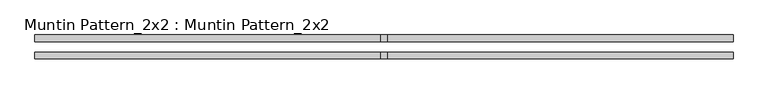
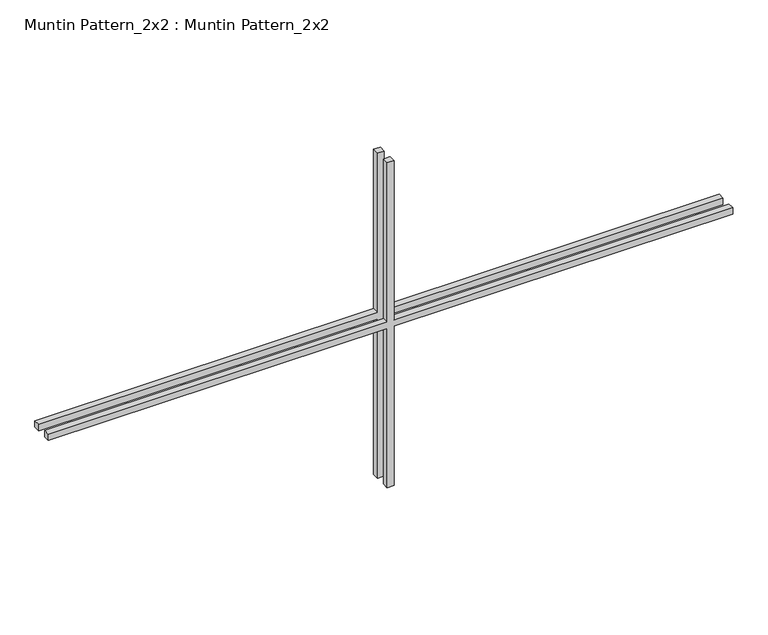
"""IFC4 building model written with IfcOpenShell, lengths in millimetres: proxy geometry, Muntin Pattern_2x2 : Muntin Pattern_2x2."""

import ifcopenshell
import ifcopenshell.guid

model = None  # the IFC model being written
_history = None  # IfcOwnerHistory: only IFC2X3 demands one
_inside = {}  # id of a spatial element -> (the spatial element, [elements in it])
_under = {}  # id of a project, library or spatial element -> (it, [spatial elements below it])
_declared = {}  # id of a project -> (the project, [libraries it declares])
_typed = {}  # id of a type object -> (the type object, [elements of that type])
_made_of = {}  # id of a material, layer set ... -> (it, [elements and type objects made of it])


def new_model(schema):
    """Start an empty IFC model of exactly this schema.

    Asked for "IFC4X3", IfcOpenShell would pick the latest addendum, in which some entities
    have other attributes; the version numbers below select the first issue.
    IFC2X3 requires an IfcOwnerHistory on every rooted entity: one is made here for all.
    """
    global model, _history
    if schema == "IFC4X3":
        model = ifcopenshell.file(schema_version=(4, 3, 0, 0))
    else:
        model = ifcopenshell.file(schema=schema)
    _inside.clear()
    _under.clear()
    _declared.clear()
    _typed.clear()
    _made_of.clear()
    _history = None
    if model.schema == "IFC2X3":
        org = make("IfcOrganization", Name="unknown")
        user = make(
            "IfcPersonAndOrganization",
            ThePerson=make("IfcPerson", FamilyName="unknown"),
            TheOrganization=org,
        )
        app = make(
            "IfcApplication",
            ApplicationDeveloper=org,
            Version="unknown",
            ApplicationFullName="unknown",
            ApplicationIdentifier="unknown",
        )
        _history = make(
            "IfcOwnerHistory",
            OwningUser=user,
            OwningApplication=app,
            ChangeAction="ADDED",
            CreationDate=0,
        )
    return model


def make(cls, **values):
    """One entity of the class cls with the attributes given. An attribute that is None is left unset."""
    return model.create_entity(
        cls, **{name: value for name, value in values.items() if value is not None}
    )


def rooted(cls, **values):
    """An entity with a GlobalId (a new one), such as an element, a storey or a relation."""
    return make(cls, GlobalId=ifcopenshell.guid.new(), OwnerHistory=_history, **values)


def si_unit(unit_type, name, prefix=None):
    """IfcSIUnit, for example si_unit("LENGTHUNIT", "METRE", prefix="MILLI")."""
    return make("IfcSIUnit", UnitType=unit_type, Prefix=prefix, Name=name)


def assignment(units):
    """IfcUnitAssignment: the units of a project."""
    return None if units is None else make("IfcUnitAssignment", Units=units)


def point(xyz):
    """IfcCartesianPoint."""
    return None if xyz is None else make("IfcCartesianPoint", Coordinates=xyz)


def direction(xyz):
    """IfcDirection."""
    return None if xyz is None else make("IfcDirection", DirectionRatios=xyz)


def frame(location, z_axis=None, x_axis=None):
    """IfcAxis2Placement3D, a coordinate frame: its origin and axes. An axis left out is left unset."""
    return make(
        "IfcAxis2Placement3D",
        Location=point(location),
        Axis=direction(z_axis),
        RefDirection=direction(x_axis),
    )


def origin():
    """The frame at (0, 0, 0) with its axes left unset."""
    return frame((0.0, 0.0, 0.0))


def place(relative_to, where):
    """IfcLocalPlacement: puts the frame where relative to a parent placement (None: the world)."""
    return make(
        "IfcLocalPlacement", PlacementRelTo=relative_to, RelativePlacement=where
    )


def context(
    kind, dimensions, precision=None, world=None, true_north=None, identifier=None
):
    """IfcGeometricRepresentationContext, for example the 3D "Model" context."""
    return make(
        "IfcGeometricRepresentationContext",
        ContextIdentifier=identifier,
        ContextType=kind,
        CoordinateSpaceDimension=dimensions,
        Precision=precision,
        WorldCoordinateSystem=world,
        TrueNorth=true_north,
    )


def project(units=None, contexts=None):
    """IfcProject with its units and contexts."""
    return rooted(
        "IfcProject",
        Name="project",
        RepresentationContexts=contexts,
        UnitsInContext=assignment(units),
    )


def spatial(cls, under=None, at=None, **own):
    """A site, building, storey or space (cls), placed at a placement, below another one or the project."""
    s = rooted(cls, ObjectPlacement=at, **own)
    if under is not None:
        _under.setdefault(under.id(), (under, []))[1].append(s)
    return s


def polyline(points):
    """IfcPolyline through the points."""
    return make("IfcPolyline", Points=[point(p) for p in points])


def outline(outer, holes=None, kind="AREA"):
    """IfcArbitraryClosedProfileDef: a profile drawn as a closed curve; with holes, ...WithVoids."""
    if holes is None:
        return make("IfcArbitraryClosedProfileDef", ProfileType=kind, OuterCurve=outer)
    return make(
        "IfcArbitraryProfileDefWithVoids",
        ProfileType=kind,
        OuterCurve=outer,
        InnerCurves=holes,
    )


def extrude(swept, where, along, depth):
    """IfcExtrudedAreaSolid: the profile swept, set in the frame where, extruded along a direction by depth."""
    return make(
        "IfcExtrudedAreaSolid",
        SweptArea=swept,
        Position=where,
        ExtrudedDirection=direction(along),
        Depth=depth,
    )


def shape(context_of_items, identifier, shape_type, items):
    """IfcShapeRepresentation: the items that make up one representation, for example the "Body"."""
    return make(
        "IfcShapeRepresentation",
        ContextOfItems=context_of_items,
        RepresentationIdentifier=identifier,
        RepresentationType=shape_type,
        Items=items,
    )


def source(mapping_origin, context_of_items, identifier, shape_type, items):
    """IfcRepresentationMap: a shape defined once, which mapped items show again and again."""
    return make(
        "IfcRepresentationMap",
        MappingOrigin=mapping_origin,
        MappedRepresentation=shape(context_of_items, identifier, shape_type, items),
    )


def transform(
    local_origin,
    x_axis=None,
    y_axis=None,
    z_axis=None,
    scale=None,
    scale2=None,
    scale3=None,
    uniform=True,
):
    """IfcCartesianTransformationOperator3D, or its non-uniform kind. x_axis, y_axis, z_axis: its Axis1, 2, 3."""
    if uniform:
        return make(
            "IfcCartesianTransformationOperator3D",
            Axis1=direction(x_axis),
            Axis2=direction(y_axis),
            LocalOrigin=point(local_origin),
            Scale=scale,
            Axis3=direction(z_axis),
        )
    return make(
        "IfcCartesianTransformationOperator3DnonUniform",
        Axis1=direction(x_axis),
        Axis2=direction(y_axis),
        LocalOrigin=point(local_origin),
        Scale=scale,
        Axis3=direction(z_axis),
        Scale2=scale2,
        Scale3=scale3,
    )


def mapped(mapping_source, mapping_target):
    """IfcMappedItem: shows the shape of a source again, moved by a transform."""
    return make(
        "IfcMappedItem", MappingSource=mapping_source, MappingTarget=mapping_target
    )


def made_of(thing, what):
    """Note that an element or type object is made of a material, layer set ...; save() writes the relation."""
    if what is not None:
        _made_of.setdefault(what.id(), (what, []))[1].append(thing)
    return thing


def element(
    cls,
    number,
    at=None,
    inside=None,
    cuts=None,
    type_object=None,
    material=None,
    context=None,
    identifier="Body",
    shape_type=None,
    held_by="IfcProductDefinitionShape",
    body=None,
    shapes=None,
    **own,
):
    """One element of the class cls, such as IfcWall. Its Tag is "e" and its number.

    at: its placement. inside: the storey or other place that contains it. cuts: it is an
    opening in that element (IfcRelVoidsElement). A single representation is given by context,
    identifier, shape_type and body (its items); several are given by shapes. held_by: the class
    of the entity that holds the representations. save() writes the other relations.
    """
    e = rooted(cls, Tag="e%d" % number, ObjectPlacement=at, **own)
    if body is not None:
        shapes = [shape(context, identifier, shape_type, body)]
    if shapes is not None:
        e.Representation = make(held_by, Representations=shapes)
    if inside is not None:
        _inside.setdefault(inside.id(), (inside, []))[1].append(e)
    if cuts is not None:
        rooted(
            "IfcRelVoidsElement", RelatingBuildingElement=cuts, RelatedOpeningElement=e
        )
    if type_object is not None:
        _typed.setdefault(type_object.id(), (type_object, []))[1].append(e)
    return made_of(e, material)


def aggregate(whole, parts):
    """IfcRelAggregates: a whole, such as a stair, and the parts it consists of."""
    return rooted("IfcRelAggregates", RelatingObject=whole, RelatedObjects=parts)


def save(model, path):
    """Write the relations noted so far, then the file.

    IfcRelAggregates (storeys below a building ...), IfcRelContainedInSpatialStructure (elements
    in a storey), IfcRelDefinesByType, IfcRelAssociatesMaterial and IfcRelDeclares: one each for
    every whole, place, type object, material and project.
    """
    for whole, parts in _under.values():
        aggregate(whole, parts)
    for where, things in _inside.values():
        rooted(
            "IfcRelContainedInSpatialStructure",
            RelatedElements=things,
            RelatingStructure=where,
        )
    for kind, things in _typed.values():
        rooted("IfcRelDefinesByType", RelatedObjects=things, RelatingType=kind)
    for what, things in _made_of.values():
        rooted("IfcRelAssociatesMaterial", RelatedObjects=things, RelatingMaterial=what)
    for by, libraries in _declared.values():
        rooted("IfcRelDeclares", RelatingContext=by, RelatedDefinitions=libraries)
    model.write(path)


def muntin_pattern_2x2_muntin_pattern_2x2_56bcf098(model_context):
    return source(origin(), model_context, "Body", "SweptSolid", [
        extrude(outline(polyline([(331.7875, -6.35), (331.7875, -647.7), (319.0875, -647.7), (319.0875, -6.35), (0.0, -6.35), (0.0, 6.35), (319.0875, 6.35), (319.0875, 647.7), (331.7875, 647.7), (331.7875, 6.35), (650.875, 6.35), (650.875, -6.35), (331.7875, -6.35)])), frame((0.0, 9.525, 0.0), z_axis=(0.0, 1.0, 0.0), x_axis=(0.0, 0.0, 1.0)), (0.0, 0.0, 1.0), 12.7),
        extrude(outline(polyline([(331.7875, -6.35), (331.7875, -647.7), (319.0875, -647.7), (319.0875, -6.35), (0.0, -6.35), (0.0, 6.35), (319.0875, 6.35), (319.0875, 647.7), (331.7875, 647.7), (331.7875, 6.35), (650.875, 6.35), (650.875, -6.35), (331.7875, -6.35)])), frame((0.0, -22.225, 0.0), z_axis=(0.0, 1.0, 0.0), x_axis=(0.0, 0.0, 1.0)), (0.0, 0.0, 1.0), 12.7),
    ])


if __name__ == "__main__":
    model = new_model("IFC4")
    model_context = context("Model", 3, world=origin())
    ifc_project = project(units=[si_unit("LENGTHUNIT", "METRE", prefix="MILLI")], contexts=[model_context])
    site = spatial("IfcSite", under=ifc_project)
    building = spatial("IfcBuilding", under=site)
    placement = place(None, origin())
    muntin_pattern_2x2_muntin_pattern_2x2_shape = muntin_pattern_2x2_muntin_pattern_2x2_56bcf098(model_context)
    element("IfcBuildingElementProxy", 1, Name="Muntin Pattern_2x2 : Muntin Pattern_2x2", ObjectType="Muntin Pattern_2x2 : Muntin Pattern_2x2", at=placement, inside=building, context=model_context, shape_type="MappedRepresentation", body=[
        mapped(muntin_pattern_2x2_muntin_pattern_2x2_shape, transform((0.0, 0.0, 0.0), x_axis=(1.0, 0.0, 0.0), y_axis=(0.0, 1.0, 0.0), z_axis=(0.0, 0.0, 1.0))),
    ])
    save(model, "model.ifc")

# Revit data of these elements
# Type "Muntin Pattern_2x2 : Muntin Pattern_2x2"
#   Width [instance default] = 4' - 0"
#   Thickness = 0' - 0 1/2"
#   Height [instance default] = 4' - 0"
#   Distance = 0' - 0 3/4"
#   Interior Material [instance default] = none
#   Exterior Material [instance default] = none
# Element 1 (IfcBuildingElementProxy, "Muntin Pattern_2x2 : Muntin Pattern_2x2")
#   Width = 4' - 3"
#   Height = 2' - 1 5/8"
#   Interior Material = Wood - Stained
#   Exterior Material = Clad - White
#   Materials on its faces: "Clad - White", "Wood - Stained"
# Materials
#   "Clad - White": class "Wood", colour RGB 242 242 238, transparency 0, Cost = 0
#   "Wood - Stained": class "Wood", colour RGB 224 178 126, transparency 0, Cost = 0
